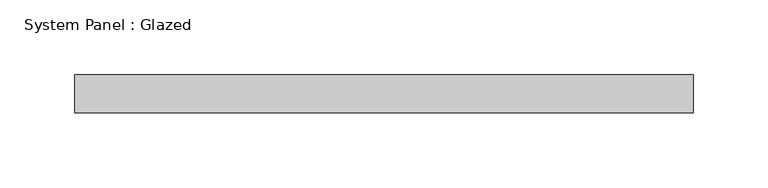
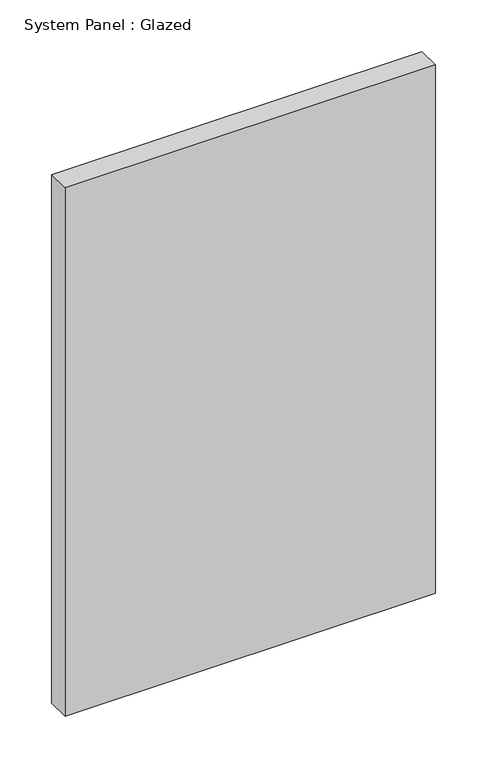
"""IFC4 building model written with IfcOpenShell, lengths in millimetres: plate geometry, System Panel : Glazed."""

from ifc_helpers import new_model, si_unit, origin, origin_with_axes, place, context, project, spatial, polyline, outline, extrude, source, transform, mapped, element, save


def system_panel_glazed_4a110745(model_context):
    return source(origin(), model_context, "Body", "SweptSolid", [
        extrude(outline(polyline([(206.3749998, 19.05), (-206.3749998, 19.05), (-206.3749998, 44.45), (206.3749998, 44.45), (206.3749998, 19.05)])), origin_with_axes(), (0.0, 0.0, 1.0), 622.3),
    ])


if __name__ == "__main__":
    model = new_model("IFC4")
    model_context = context("Model", 3, world=origin())
    ifc_project = project(units=[si_unit("LENGTHUNIT", "METRE", prefix="MILLI")], contexts=[model_context])
    site = spatial("IfcSite", under=ifc_project)
    building = spatial("IfcBuilding", under=site)
    placement = place(None, origin())
    system_panel_glazed_shape = system_panel_glazed_4a110745(model_context)
    element("IfcPlate", 1, ObjectType="System Panel : Glazed", at=placement, inside=building, context=model_context, shape_type="MappedRepresentation", body=[
        mapped(system_panel_glazed_shape, transform((0.0, 0.0, 0.0), x_axis=(1.0, 0.0, 0.0), y_axis=(0.0, 1.0, 0.0), z_axis=(0.0, 0.0, 1.0))),
    ])
    save(model, "model.ifc")

# Revit data of these elements
# Element 1 (IfcPlate, "System Panel : Glazed")
#   Materials on its faces: "Glass"
# Materials
#   "Glass": class "Glass", colour RGB 0 128 192, transparency 0.75
